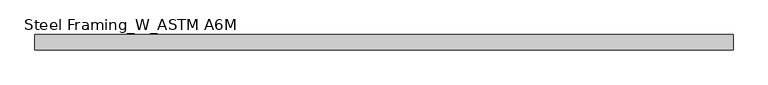
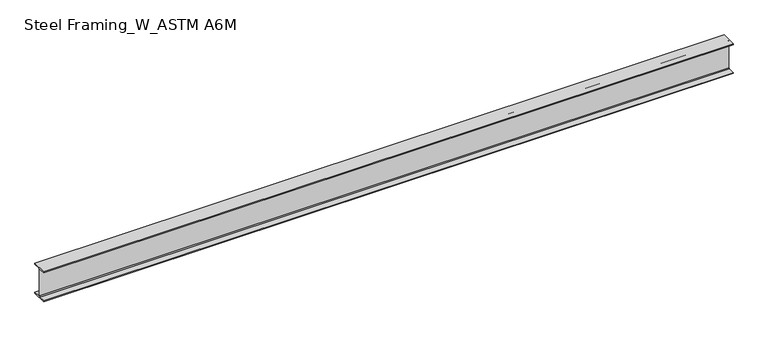
"""IFC4 building model written with IfcOpenShell, lengths in millimetres: beam geometry, Steel Framing_W_ASTM A6M : H_SB_AR_S02_W360x51_G3."""

from ifc_helpers import new_model, si_unit, point, frame, frame_2d, origin, place, context, project, spatial, polyline, circle_curve, trimmed, segment, composite_curve, outline, extrude, source, transform, mapped, element, save


def steel_framing_w_astm_a6m_becc2698(model_context):
    return source(origin(), model_context, "Body", "SweptSolid", [
        extrude(outline(composite_curve([segment(polyline([(85.5, -166.4), (85.5, -178.0), (-85.5, -178.0), (-85.5, -166.4), (-13.72, -166.4)]), True, "CONTINUOUS"), segment(trimmed(circle_curve(frame_2d((-13.72, -156.3)), 10.1), [point((-13.72, -166.4))], [point((-3.62, -156.3))], True, "CARTESIAN"), True, "CONTINUOUS"), segment(polyline([(-3.62, -156.3), (-3.62, 156.3)]), True, "CONTINUOUS"), segment(trimmed(circle_curve(frame_2d((-13.72, 156.3)), 10.1), [point((-3.62, 156.3))], [point((-13.72, 166.4))], True, "CARTESIAN"), True, "CONTINUOUS"), segment(polyline([(-13.72, 166.4), (-85.5, 166.4), (-85.5, 178.0), (85.5, 178.0), (85.5, 166.4), (13.72, 166.4)]), True, "CONTINUOUS"), segment(trimmed(circle_curve(frame_2d((13.72, 156.3)), 10.1), [point((13.72, 166.4))], [point((3.62, 156.3))], True, "CARTESIAN"), True, "CONTINUOUS"), segment(polyline([(3.62, 156.3), (3.62, -156.3)]), True, "CONTINUOUS"), segment(trimmed(circle_curve(frame_2d((13.72, -156.3)), 10.1), [point((3.62, -156.3))], [point((13.72, -166.4))], True, "CARTESIAN"), True, "CONTINUOUS"), segment(polyline([(13.72, -166.4), (85.5, -166.4)]), True, "CONTINUOUS")], self_intersect=False)), frame((-3884.3, 0.0, 0.0), z_axis=(1.0, 0.0, 0.0), x_axis=(0.0, 1.0, 0.0)), (0.0, 0.0, 1.0), 7768.6),
    ])


if __name__ == "__main__":
    model = new_model("IFC4")
    model_context = context("Model", 3, world=origin())
    ifc_project = project(units=[si_unit("LENGTHUNIT", "METRE", prefix="MILLI")], contexts=[model_context])
    site = spatial("IfcSite", under=ifc_project)
    building = spatial("IfcBuilding", under=site)
    placement = place(None, origin())
    steel_framing_w_astm_a6m_shape = steel_framing_w_astm_a6m_becc2698(model_context)
    element("IfcBeam", 1, ObjectType="Steel Framing_W_ASTM A6M : H_SB_AR_S02_W360x51_G3", at=placement, inside=building, context=model_context, shape_type="MappedRepresentation", body=[
        mapped(steel_framing_w_astm_a6m_shape, transform((0.0, 0.0, 0.0), x_axis=(1.0, 0.0, 0.0), y_axis=(0.0, 1.0, 0.0), z_axis=(0.0, 0.0, 1.0))),
    ])
    save(model, "model.ifc")

# Revit data of these elements
# Type "Steel Framing_W_ASTM A6M : H_SB_AR_S02_W360x51_G3"
#   Type Mark = "G3"
#   Section Name Key = "W14x34"
#   Width = 17.1 cm
#   Web Thickness = 0.724 cm
#   Web Fillet = 1.01 cm
#   Warping Constant = 287000.0 cm⁶
#   Torsional Moment of Inertia = 23.70 cm⁴
#   Section Area = 64.5 cm²
#   Plastic Modulus weak axis = 174.0 cm³
#   Plastic Modulus strong axis = 895.0 cm³
#   Perimeter = 1.36 m²/m
#   Nominal Weight = 51.00 kgf/m
#   Moment of Inertia weak axis = 970.00 cm⁴
#   Moment of Inertia strong axis = 14200.00 cm⁴
#   Height = 35.6 cm
#   Flange Thickness = 1.16 cm
#   Elastic Modulus weak axis = 113.0 cm³
#   Elastic Modulus strong axis = 796.0 cm³
#   Centroid Vertical = 17.8 cm
#   Centroid Horizontal = 8.55 cm
#   Length [instance default] = 1500 mm
#   Structural Material [instance default] = Steel, 45-345
#   Bolt Spacing = 0
#   Assembly Code = ""
# Element 1 (IfcBeam, "Steel Framing_W_ASTM A6M : H_SB_AR_S02_W360x51_G3")
#   Materials on its faces: "Steel, 45-345"
# Materials
#   "Steel, 45-345": class "Metal", colour RGB 189 187 185, transparency 0, Description = "Steel 345 MPa", Cost = 0
